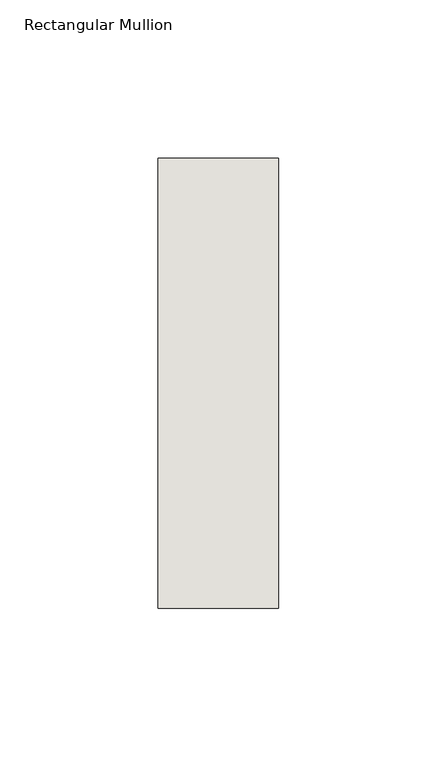
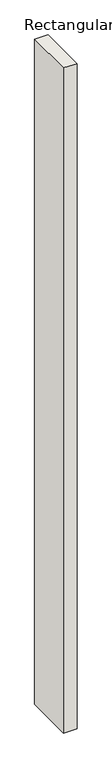
"""IFC4 building model written with IfcOpenShell, lengths in millimetres: wall geometry, Rectangular Mullion : NLRS_21_CWM_hsb-regel 38x142_gen_rsf."""

from ifc_helpers import new_model, si_unit, frame, origin, place, context, project, spatial, polyline, outline, extrude, source, transform, mapped, element, save


def rectangular_mullion_a27e35f8(model_context):
    return source(origin(), model_context, "Body", "SweptSolid", [
        extrude(outline(polyline([(19.0, -71.0), (-19.0, -71.0), (-19.0, 71.0), (19.0, 71.0), (19.0, -71.0)])), frame((0.0, 0.0, -2000.0), z_axis=(0.0, 0.0, 1.0), x_axis=(1.0, 0.0, 0.0)), (0.0, 0.0, 1.0), 2000.0),
    ])


if __name__ == "__main__":
    model = new_model("IFC4")
    model_context = context("Model", 3, world=origin())
    ifc_project = project(units=[si_unit("LENGTHUNIT", "METRE", prefix="MILLI")], contexts=[model_context])
    site = spatial("IfcSite", under=ifc_project)
    building = spatial("IfcBuilding", under=site)
    placement = place(None, origin())
    rectangular_mullion_shape = rectangular_mullion_a27e35f8(model_context)
    element("IfcWall", 1, ObjectType="Rectangular Mullion : NLRS_21_CWM_hsb-regel 38x142_gen_rsf", at=placement, inside=building, context=model_context, shape_type="MappedRepresentation", body=[
        mapped(rectangular_mullion_shape, transform((0.0, 0.0, 0.0), x_axis=(1.0, 0.0, 0.0), y_axis=(0.0, 1.0, 0.0), z_axis=(0.0, 0.0, 1.0))),
    ])
    save(model, "model.ifc")

# Revit data of these elements
# Type "Rectangular Mullion : NLRS_21_CWM_hsb-regel 38x142_gen_rsf"
#   Type IfcGUID = "07M7mRoiH1CR8m_RSKIwpF"
#   Assembly Code = "21.10"
#   IfcExportAs = "IfcWall"
#   built-in parameter 1007322 = 0.465879 (stored number, unit not read)
#   built-in parameter 1007321 = 0.062336 (stored number, unit not read)
#   built-in parameter 1007320 = 0.062336 (stored number, unit not read)
# Element 1 (IfcWall, "Rectangular Mullion : NLRS_21_CWM_hsb-regel 38x142_gen_rsf")
#   Materials on its faces: "NLRS_i2_hout naaldhout vuren_gen_rsf"
# Materials
#   "NLRS_i2_hout naaldhout vuren_gen_rsf": class "I - Hout", colour RGB 234 199 147, transparency 0, Keynote = "i2", Manufacturer = "Revit Standards Foundation", URL = "www.revitstandards.org", Description = "hout vuren", Cost = 0
